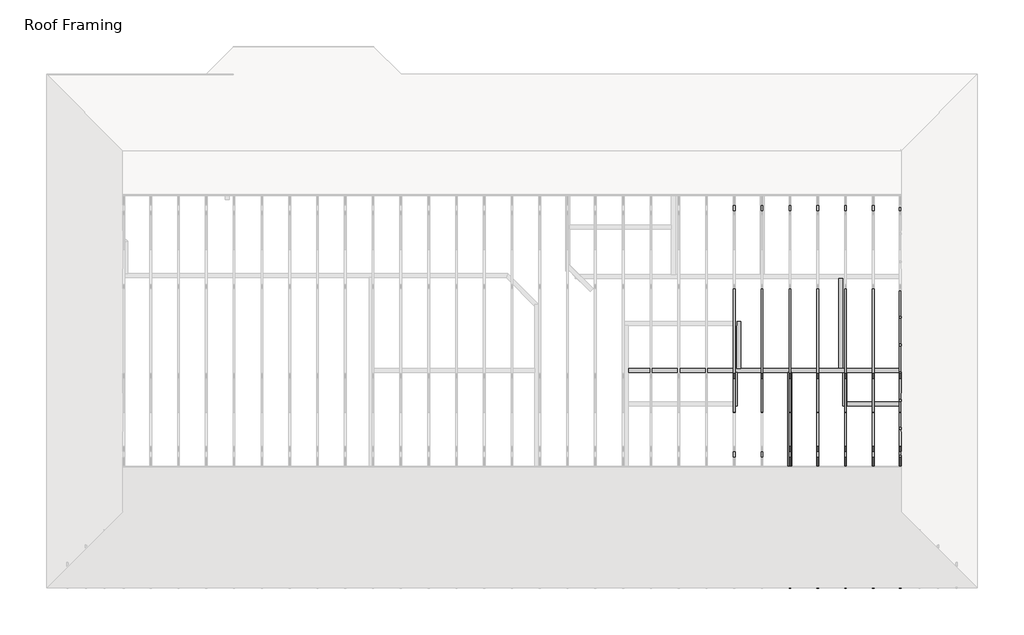
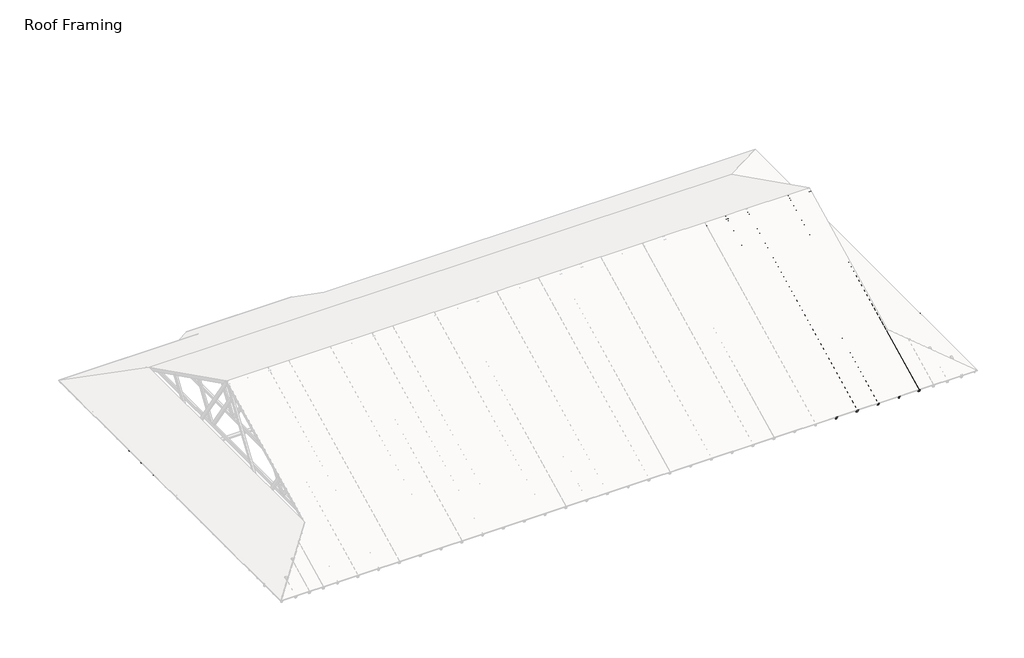
# One storey, part 4 of 7: 53 beams, 12 members.
# Revit data of these elements (continued)
# Elements 54, 55, 56, 57, 58, 59, 60, 61, 62, 63, 64, 65 (IfcMember, "Dimension Lumber : 2x4 Truss")
#   Comments = ""
#   Structural Material = Douglas Fir #2
#   Phase Created = New Construction
#   Materials on its faces: "Douglas Fir #2"
# Materials
#   "Softwood, Lumber": class "Wood", colour RGB 223 192 134, transparency 0, Description = "Pinus Echinata", Cost = 0
#   "Douglas Fir #2": class "Wood", colour RGB 223 192 134, transparency 0, Description = "Pinus Echinata", Cost = 0
